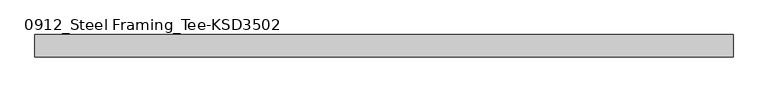
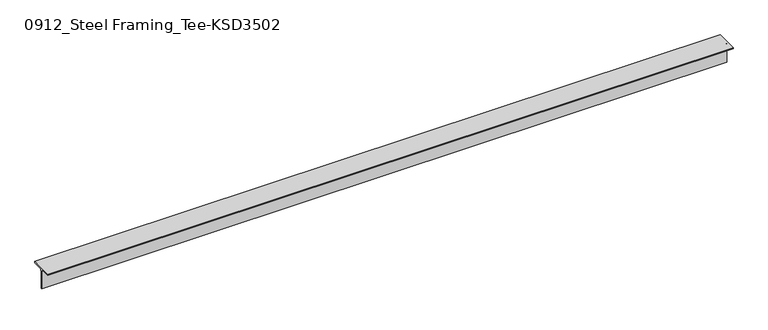
"""IFC4 building model written with IfcOpenShell, lengths in millimetres: member geometry, 0912_Steel Framing_Tee-KSD3502 : H_SB_ASB_CT-150x150x6.5x9."""

from ifc_helpers import new_model, si_unit, point, frame, frame_2d, origin, place, context, project, spatial, polyline, circle_curve, trimmed, segment, composite_curve, outline, extrude, source, transform, mapped, element, save


def member_0912_steel_framing_tee_ksd3502_626917b6(model_context):
    return source(origin(), model_context, "Body", "SweptSolid", [
        extrude(outline(composite_curve([segment(polyline([(-75.0, 75.0), (75.0, 75.0), (75.0, 66.0), (16.25, 66.0)]), True, "CONTINUOUS"), segment(trimmed(circle_curve(frame_2d((16.25, 53.0)), 13.0), [point((16.25, 66.0))], [point((3.25, 53.0))], True, "CARTESIAN"), True, "CONTINUOUS"), segment(polyline([(3.25, 53.0), (3.25, -75.0), (-3.25, -75.0), (-3.25, 53.0)]), True, "CONTINUOUS"), segment(trimmed(circle_curve(frame_2d((-16.25, 53.0)), 13.0), [point((-3.25, 53.0))], [point((-16.25, 66.0))], True, "CARTESIAN"), True, "CONTINUOUS"), segment(polyline([(-16.25, 66.0), (-75.0, 66.0), (-75.0, 75.0)]), True, "CONTINUOUS")], self_intersect=False)), frame((-2303.1, 0.0, 0.0), z_axis=(1.0, 0.0, 0.0), x_axis=(0.0, 1.0, 0.0)), (0.0, 0.0, 1.0), 4645.3),
    ])


if __name__ == "__main__":
    model = new_model("IFC4")
    model_context = context("Model", 3, world=origin())
    ifc_project = project(units=[si_unit("LENGTHUNIT", "METRE", prefix="MILLI")], contexts=[model_context])
    site = spatial("IfcSite", under=ifc_project)
    building = spatial("IfcBuilding", under=site)
    placement = place(None, origin())
    member_0912_steel_framing_tee_ksd3502_shape = member_0912_steel_framing_tee_ksd3502_626917b6(model_context)
    element("IfcMember", 1, ObjectType="0912_Steel Framing_Tee-KSD3502 : H_SB_ASB_CT-150x150x6.5x9", at=placement, inside=building, context=model_context, shape_type="MappedRepresentation", body=[
        mapped(member_0912_steel_framing_tee_ksd3502_shape, transform((0.0, 0.0, 0.0), x_axis=(1.0, 0.0, 0.0), y_axis=(0.0, 1.0, 0.0), z_axis=(0.0, 0.0, 1.0))),
    ])
    save(model, "model.ifc")

# Revit data of these elements
# Type "0912_Steel Framing_Tee-KSD3502 : H_SB_ASB_CT-150x150x6.5x9"
#   H_WM Code_1 = "S01AA003-00001 | Main Steel Structure Fabrication Work | Shelter/Building | Light Steel - Standard (30KG/M>Weight) | Material: (   )"
#   H_WM Code_2 = "S03AA029-00001 | Main Steel Structure Erection Work | Shelter/Building | Light Steel (30KG/M>Weight) | Material: (   )"
#   H_WM Code_3 = "S01AA010-00001 | Main Steel Structure Fabrication Work | Shelter/Building | Steel Painting/Coating | for Non-Fireproofed Steel Surface, Surface Preparation, Primer, Second & Final Coat | Material: (   )"
#   H_Q'ty Cal Type Tag = "SB-Q2"
#   Width = 15.0 cm
#   Web Thickness = 0.65 cm
#   Web Fillet = 1.3 cm
#   Section Area = 23.39 cm²
#   Perimeter = 0.60 m²/m
#   Nominal Weight = 18.40 kgf/m
#   Height = 15.0 cm
#   Flange Thickness = 0.9 cm
#   Centroid Vertical = 7.5 cm
#   Centroid Horizontal = 7.5 cm
#   Length [instance default] = 1.5000 m
#   Structural Material [instance default] = Steel, 45-345
#   Warping Constant = (empty or 0)
#   Torsional Moment of Inertia = 0
#   Section Name Key = ""
#   Plastic Modulus weak axis = 0
#   Plastic Modulus strong axis = 0
#   Moment of Inertia weak axis = 0
#   Moment of Inertia strong axis = 0
#   Elastic Modulus weak axis = 0
#   Elastic Modulus strong axis = 0
#   Bolt Spacing = 0
#   Assembly Code = ""
# Element 1 (IfcMember, "0912_Steel Framing_Tee-KSD3502 : H_SB_ASB_CT-150x150x6.5x9")
#   Structural Material = none
# Materials
#   "Steel, 45-345": class "Metal", colour RGB 189 187 185, transparency 0, Description = "Steel 345 MPa", Cost = 0
